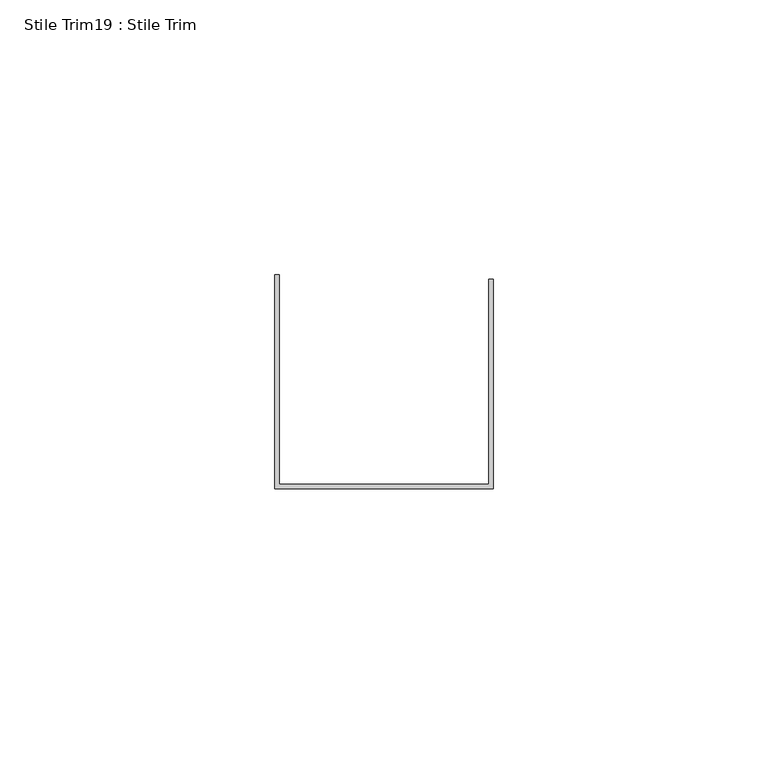
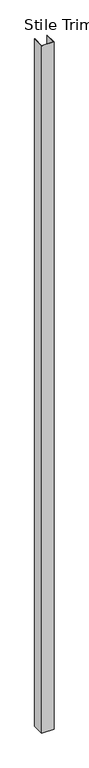
"""IFC4 building model written with IfcOpenShell, lengths in millimetres: proxy geometry, Stile Trim19 : Stile Trim."""

from ifc_helpers import new_model, si_unit, frame, origin, place, context, project, spatial, polyline, outline, extrude, source, transform, mapped, element, save


def stile_trim19_stile_trim_35358b3a(model_context):
    return source(origin(), model_context, "Body", "SweptSolid", [
        extrude(outline(polyline([(587327.0060739, -532878.2537841), (587327.0060739, -532839.3663841), (587327.7934739, -532839.3663841), (587327.7934739, -532877.4663841), (587365.8934739, -532877.4663841), (587365.8934739, -532840.1537841), (587366.6808739, -532840.1537841), (587366.6808739, -532878.2537841), (587327.0060739, -532878.2537841)])), frame((0.0, 0.0, 50.8), z_axis=(0.0, 0.0, 1.0), x_axis=(1.0, 0.0, 0.0)), (0.0, 0.0, 1.0), 2350.3929688),
    ])


if __name__ == "__main__":
    model = new_model("IFC4")
    model_context = context("Model", 3, world=origin())
    ifc_project = project(units=[si_unit("LENGTHUNIT", "METRE", prefix="MILLI")], contexts=[model_context])
    site = spatial("IfcSite", under=ifc_project)
    building = spatial("IfcBuilding", under=site)
    placement = place(None, origin())
    stile_trim19_stile_trim_shape = stile_trim19_stile_trim_35358b3a(model_context)
    element("IfcBuildingElementProxy", 1, Name="Stile Trim19 : Stile Trim", ObjectType="Stile Trim19 : Stile Trim", at=placement, inside=building, context=model_context, shape_type="MappedRepresentation", body=[
        mapped(stile_trim19_stile_trim_shape, transform((0.0, 0.0, 0.0), x_axis=(1.0, 0.0, 0.0), y_axis=(0.0, 1.0, 0.0), z_axis=(0.0, 0.0, 1.0))),
    ])
    save(model, "model.ifc")

# Revit data of these elements
# Element 1 (IfcBuildingElementProxy, "Stile Trim19 : Stile Trim")
#   Materials on its faces: "EDGE TRIM BY MTL PANEL MFR."
# Materials
#   "EDGE TRIM BY MTL PANEL MFR.": class "Generic", colour RGB 239 242 240, transparency 0, Cost = 0
